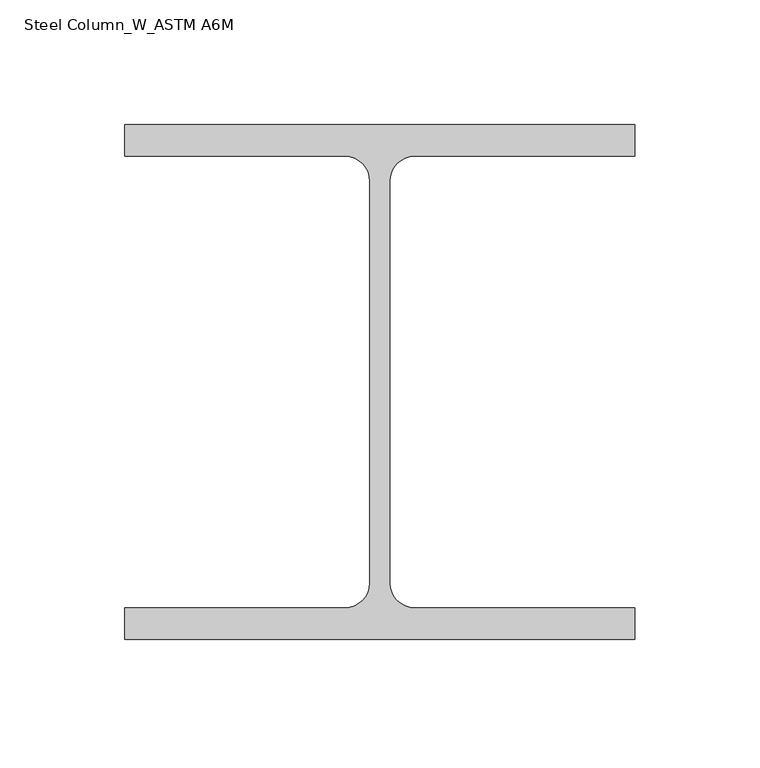
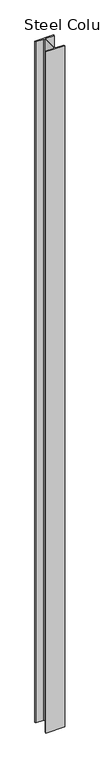
"""IFC4 building model written with IfcOpenShell, lengths in millimetres: column geometry, Steel Column_W_ASTM A6M : H_SC_AR_S01_W200x52_C2."""

from ifc_helpers import new_model, si_unit, point, frame, frame_2d, origin, place, context, project, spatial, polyline, circle_curve, trimmed, segment, composite_curve, outline, extrude, source, transform, mapped, element, save


def steel_column_w_astm_a6m_aefabb8c(model_context):
    return source(origin(), model_context, "Body", "SweptSolid", [
        extrude(outline(composite_curve([segment(polyline([(102.0, 103.0), (102.0, 90.4), (13.935, 90.4)]), True, "CONTINUOUS"), segment(trimmed(circle_curve(frame_2d((13.935, 80.4)), 10.0), [point((13.935, 90.4))], [point((3.935, 80.4))], True, "CARTESIAN"), True, "CONTINUOUS"), segment(polyline([(3.935, 80.4), (3.935, -80.4)]), True, "CONTINUOUS"), segment(trimmed(circle_curve(frame_2d((13.935, -80.4)), 10.0), [point((3.935, -80.4))], [point((13.935, -90.4))], True, "CARTESIAN"), True, "CONTINUOUS"), segment(polyline([(13.935, -90.4), (102.0, -90.4), (102.0, -103.0), (-102.0, -103.0), (-102.0, -90.4), (-13.935, -90.4)]), True, "CONTINUOUS"), segment(trimmed(circle_curve(frame_2d((-13.935, -80.4)), 10.0), [point((-13.935, -90.4))], [point((-3.935, -80.4))], True, "CARTESIAN"), True, "CONTINUOUS"), segment(polyline([(-3.935, -80.4), (-3.935, 80.4)]), True, "CONTINUOUS"), segment(trimmed(circle_curve(frame_2d((-13.935, 80.4)), 10.0), [point((-3.935, 80.4))], [point((-13.935, 90.4))], True, "CARTESIAN"), True, "CONTINUOUS"), segment(polyline([(-13.935, 90.4), (-102.0, 90.4), (-102.0, 103.0), (102.0, 103.0)]), True, "CONTINUOUS")], self_intersect=False)), frame((0.0, 0.0, -7305.1756499), z_axis=(0.0, 0.0, 1.0), x_axis=(1.0, 0.0, 0.0)), (0.0, 0.0, 1.0), 7825.0),
    ])


if __name__ == "__main__":
    model = new_model("IFC4")
    model_context = context("Model", 3, world=origin())
    ifc_project = project(units=[si_unit("LENGTHUNIT", "METRE", prefix="MILLI")], contexts=[model_context])
    site = spatial("IfcSite", under=ifc_project)
    building = spatial("IfcBuilding", under=site)
    placement = place(None, origin())
    steel_column_w_astm_a6m_shape = steel_column_w_astm_a6m_aefabb8c(model_context)
    element("IfcColumn", 1, ObjectType="Steel Column_W_ASTM A6M : H_SC_AR_S01_W200x52_C2", at=placement, inside=building, context=model_context, shape_type="MappedRepresentation", body=[
        mapped(steel_column_w_astm_a6m_shape, transform((0.0, 0.0, 0.0), x_axis=(1.0, 0.0, 0.0), y_axis=(0.0, 1.0, 0.0), z_axis=(0.0, 0.0, 1.0))),
    ])
    save(model, "model.ifc")

# Revit data of these elements
# Type "Steel Column_W_ASTM A6M : H_SC_AR_S01_W200x52_C2"
#   Section Name Key = "W8x35"
#   Width = 20.4 cm
#   Web Thickness = 0.787 cm
#   Web Fillet = 1.0 cm
#   Warping Constant = 166000.0 cm⁶
#   Torsional Moment of Inertia = 32.00 cm⁴
#   Section Area = 66.5 cm²
#   Plastic Modulus weak axis = 264.0 cm³
#   Plastic Modulus strong axis = 569.0 cm³
#   Perimeter = 1.19 m²/m
#   Nominal Weight = 52.00 kgf/m
#   Moment of Inertia weak axis = 1770.00 cm⁴
#   Moment of Inertia strong axis = 5290.00 cm⁴
#   Height = 20.6 cm
#   Flange Thickness = 1.26 cm
#   Elastic Modulus weak axis = 174.0 cm³
#   Elastic Modulus strong axis = 511.0 cm³
#   Centroid Vertical = 10.3 cm
#   Centroid Horizontal = 10.2 cm
#   Structural Material [instance default] = Steel, 45-345
#   Bolt Spacing = 0
#   Assembly Code = ""
# Element 1 (IfcColumn, "Steel Column_W_ASTM A6M : H_SC_AR_S01_W200x52_C2")
#   Structural Material = Steel ASTM A992 GRADE 50
#   Materials on its faces: "Steel ASTM A992 GRADE 50"
# Materials
#   "Steel, 45-345": class "Metal", colour RGB 189 187 185, transparency 0, Description = "Steel 345 MPa", Cost = 0
#   "Steel ASTM A992 GRADE 50": class "Metal", colour RGB 120 120 120, transparency 0, Description = "Structural steel 50ksi", Cost = 0
